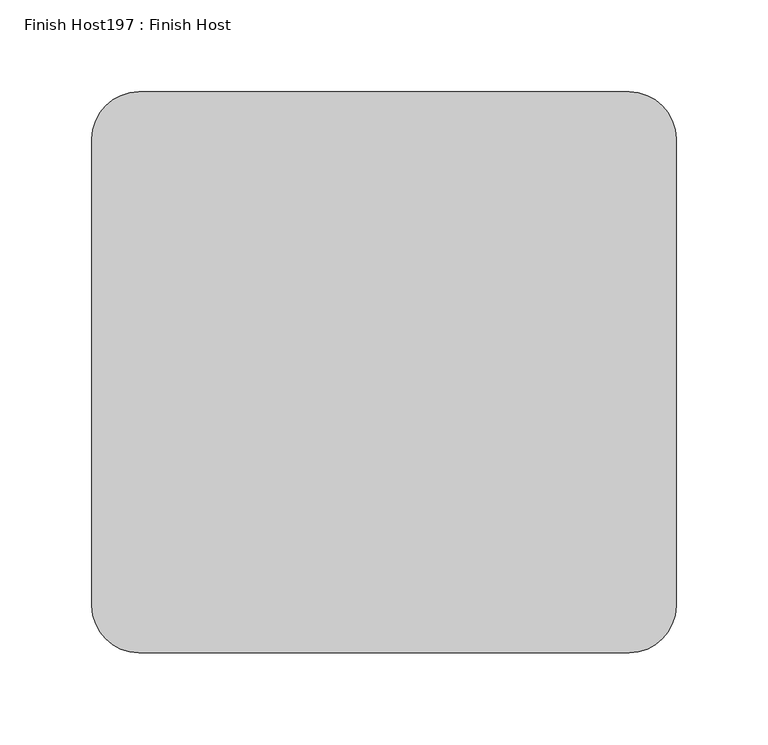
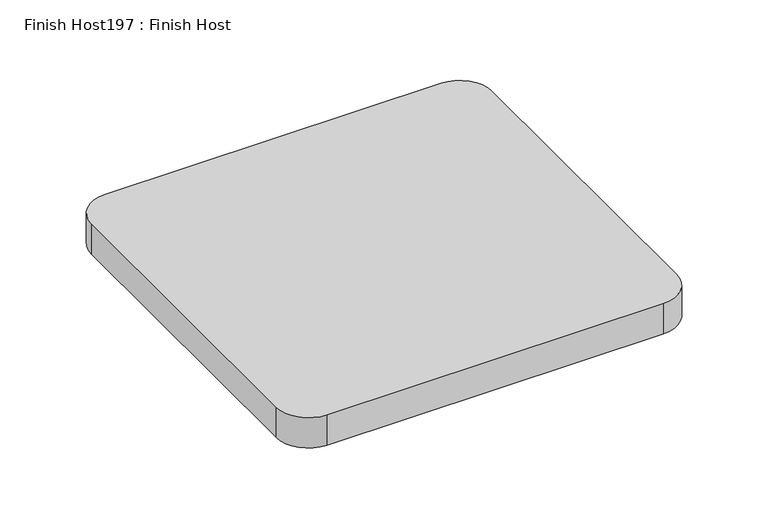
"""IFC4 building model written with IfcOpenShell, lengths in millimetres: proxy geometry, Finish Host197 : Finish Host."""

from ifc_helpers import new_model, si_unit, point, frame_2d, origin, origin_with_axes, place, context, project, spatial, polyline, circle_curve, trimmed, segment, composite_curve, outline, extrude, source, transform, mapped, element, save


def finish_host197_finish_host_85495732(model_context):
    return source(origin(), model_context, "Body", "SweptSolid", [
        extrude(outline(composite_curve([segment(polyline([(701.4157184, 3462.3960864), (701.4157184, 3716.3960864)]), True, "CONTINUOUS"), segment(trimmed(circle_curve(frame_2d((726.8157184, 3716.3960864)), 25.4), [point((701.4157184, 3716.3960864))], [point((726.8157184, 3741.7960864))], False, "CARTESIAN"), True, "CONTINUOUS"), segment(polyline([(726.8157184, 3741.7960864), (993.5157184, 3741.7960864)]), True, "CONTINUOUS"), segment(trimmed(circle_curve(frame_2d((993.5157184, 3716.3960864)), 25.4), [point((993.5157184, 3741.7960864))], [point((1018.9157184, 3716.3960864))], False, "CARTESIAN"), True, "CONTINUOUS"), segment(polyline([(1018.9157184, 3716.3960864), (1018.9157184, 3462.3960864)]), True, "CONTINUOUS"), segment(trimmed(circle_curve(frame_2d((993.5157184, 3462.3960864)), 25.4), [point((1018.9157184, 3462.3960864))], [point((993.5157184, 3436.9960864))], False, "CARTESIAN"), True, "CONTINUOUS"), segment(polyline([(993.5157184, 3436.9960864), (726.8157184, 3436.9960864)]), True, "CONTINUOUS"), segment(trimmed(circle_curve(frame_2d((726.8157184, 3462.3960864)), 25.4), [point((726.8157184, 3436.9960864))], [point((701.4157184, 3462.3960864))], False, "CARTESIAN"), True, "CONTINUOUS")], self_intersect=False)), origin_with_axes(), (0.0, 0.0, 1.0), 25.4),
    ])


if __name__ == "__main__":
    model = new_model("IFC4")
    model_context = context("Model", 3, world=origin())
    ifc_project = project(units=[si_unit("LENGTHUNIT", "METRE", prefix="MILLI")], contexts=[model_context])
    site = spatial("IfcSite", under=ifc_project)
    building = spatial("IfcBuilding", under=site)
    placement = place(None, origin())
    finish_host197_finish_host_shape = finish_host197_finish_host_85495732(model_context)
    element("IfcBuildingElementProxy", 1, Name="Finish Host197 : Finish Host", ObjectType="Finish Host197 : Finish Host", at=placement, inside=building, context=model_context, shape_type="MappedRepresentation", body=[
        mapped(finish_host197_finish_host_shape, transform((0.0, 0.0, 0.0), x_axis=(1.0, 0.0, 0.0), y_axis=(0.0, 1.0, 0.0), z_axis=(0.0, 0.0, 1.0))),
    ])
    save(model, "model.ifc")

# Revit data of these elements
# Type "Finish Host197 : Finish Host"
#   Countertop Material = Fabric - Teknion - W418 - Wales - Newbridge
# Element 1 (IfcBuildingElementProxy, "Finish Host197 : Finish Host")
#   Materials on its faces: "Fabric - Teknion - W418 - Wales - Newbridge"
# Materials
#   "Fabric - Teknion - W418 - Wales - Newbridge": class "Fabric", colour RGB 49 14 23, transparency 0, Model = "W418", Manufacturer = "Teknion Studio", URL = "http://www.teknionstudio.com/", Description = "Newbridge Wales", Cost = 0
